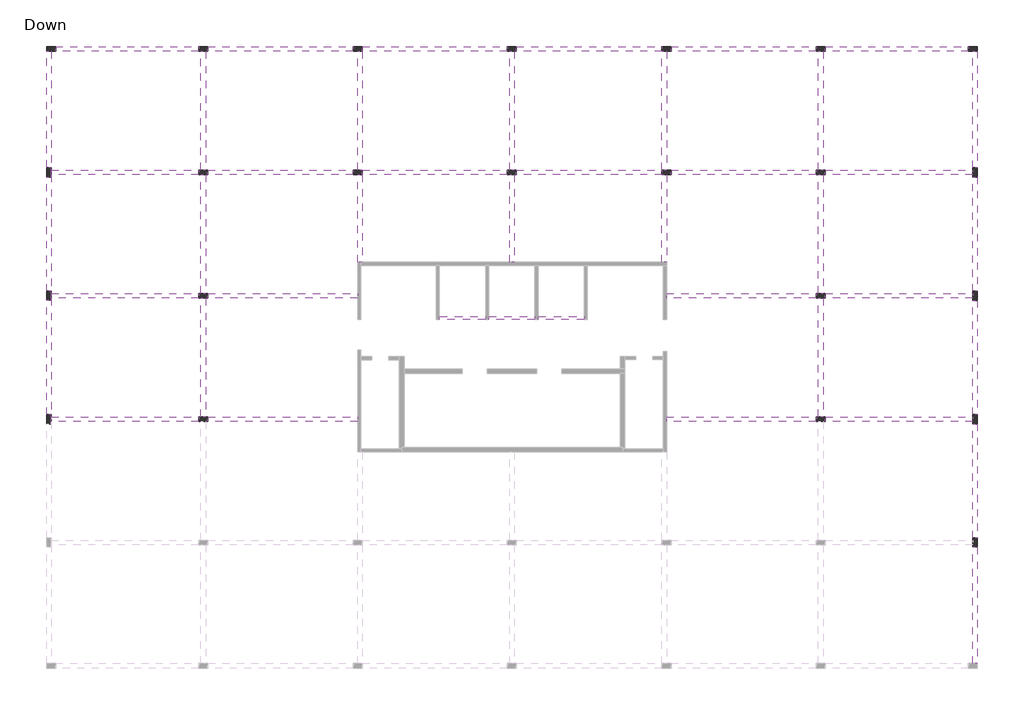
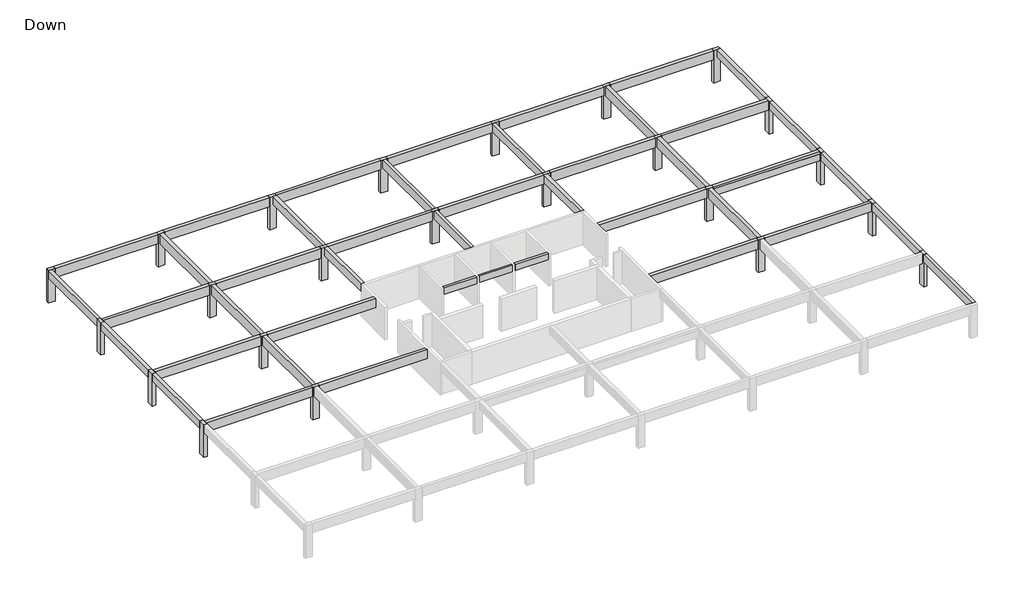
# One storey, part 2 of 2: 43 beams, 23 columns.
# Revit data of these elements (continued)
# Element 19 (IfcBeam, "Concrete Rectengular Beam : 30/85") (continued)
#   Comments = ""
#   Mark = "B27"
#   SOFiSTiK_AMG_Comments = ""
#   SOFiSTiK_AMG_Scheduled = yes
#   SOFiSTiK_AMG_Adjusted = yes
#   Structural Material = Concrete
#   Phase Created = New Construction
#   Materials on its faces: "Concrete"
# Element 20 (IfcBeam, "Concrete Rectengular Beam : 30/85")
#   Comments = ""
#   Mark = "B28"
#   SOFiSTiK_AMG_Comments = ""
#   SOFiSTiK_AMG_Scheduled = yes
#   SOFiSTiK_AMG_Adjusted = yes
#   Structural Material = Concrete
#   Phase Created = New Construction
#   Materials on its faces: "Concrete"
# Element 21 (IfcBeam, "Concrete Rectengular Beam : 30/85")
#   Comments = ""
#   Mark = "B29"
#   SOFiSTiK_AMG_Comments = ""
#   SOFiSTiK_AMG_Scheduled = yes
#   SOFiSTiK_AMG_Adjusted = yes
#   Structural Material = Concrete
#   Phase Created = New Construction
#   Materials on its faces: "Concrete"
# Element 22 (IfcBeam, "Concrete Rectengular Beam : 30/85")
#   Comments = ""
#   Mark = "B30"
#   SOFiSTiK_AMG_Comments = ""
#   SOFiSTiK_AMG_Scheduled = yes
#   SOFiSTiK_AMG_Adjusted = yes
#   Structural Material = Concrete
#   Phase Created = New Construction
#   Materials on its faces: "Concrete"
# Element 23 (IfcBeam, "Concrete Rectengular Beam : 30/85")
#   Comments = ""
#   Mark = "B31"
#   SOFiSTiK_AMG_Comments = ""
#   SOFiSTiK_AMG_Scheduled = yes
#   SOFiSTiK_AMG_Adjusted = yes
#   Structural Material = Concrete
#   Phase Created = New Construction
#   Materials on its faces: "Concrete"
# Element 24 (IfcBeam, "Concrete Rectengular Beam : 30/85")
#   Comments = ""
#   Mark = "B38"
#   SOFiSTiK_AMG_Comments = ""
#   SOFiSTiK_AMG_Scheduled = yes
#   SOFiSTiK_AMG_Adjusted = yes
#   Structural Material = Concrete
#   Phase Created = New Construction
#   Materials on its faces: "Concrete"
# Element 25 (IfcBeam, "Concrete Rectengular Beam : 30/85")
#   Comments = ""
#   Mark = "B39"
#   SOFiSTiK_AMG_Comments = ""
#   SOFiSTiK_AMG_Scheduled = yes
#   SOFiSTiK_AMG_Adjusted = yes
#   Structural Material = Concrete
#   Phase Created = New Construction
#   Materials on its faces: "Concrete"
# Element 26 (IfcBeam, "Concrete Rectengular Beam : 30/85")
#   Comments = ""
#   Mark = "B40"
#   SOFiSTiK_AMG_Comments = ""
#   SOFiSTiK_AMG_Scheduled = yes
#   SOFiSTiK_AMG_Adjusted = yes
#   Structural Material = Concrete
#   Phase Created = New Construction
#   Materials on its faces: "Concrete"
# Element 27 (IfcBeam, "Concrete Rectengular Beam : 30/85")
#   Comments = ""
#   Mark = "B41"
#   SOFiSTiK_AMG_Comments = ""
#   SOFiSTiK_AMG_Scheduled = yes
#   SOFiSTiK_AMG_Adjusted = yes
#   Structural Material = Concrete
#   Phase Created = New Construction
#   Materials on its faces: "Concrete"
# Element 28 (IfcBeam, "Concrete Rectengular Beam : 30/85")
#   Comments = ""
#   Mark = "B42"
#   SOFiSTiK_AMG_Comments = ""
#   SOFiSTiK_AMG_Scheduled = yes
#   SOFiSTiK_AMG_Adjusted = yes
#   Structural Material = Concrete
#   Phase Created = New Construction
#   Materials on its faces: "Concrete"
# Element 29 (IfcBeam, "Concrete Rectengular Beam : 30/85")
#   Comments = ""
#   Mark = "B43"
#   SOFiSTiK_AMG_Comments = ""
#   SOFiSTiK_AMG_Scheduled = yes
#   SOFiSTiK_AMG_Adjusted = yes
#   Structural Material = Concrete
#   Phase Created = New Construction
#   Materials on its faces: "Concrete"
# Element 30 (IfcBeam, "Concrete Rectengular Beam : 30/85")
#   Comments = ""
#   Mark = "B44"
#   SOFiSTiK_AMG_Comments = ""
#   SOFiSTiK_AMG_Scheduled = yes
#   SOFiSTiK_AMG_Adjusted = yes
#   Structural Material = Concrete
#   Phase Created = New Construction
#   Materials on its faces: "Concrete"
# Element 31 (IfcBeam, "Concrete Rectengular Beam : 30/85")
#   Comments = ""
#   Mark = "B45"
#   SOFiSTiK_AMG_Comments = ""
#   SOFiSTiK_AMG_Scheduled = yes
#   SOFiSTiK_AMG_Adjusted = yes
#   Structural Material = Concrete
#   Phase Created = New Construction
#   Materials on its faces: "Concrete"
# Element 32 (IfcBeam, "Concrete Rectengular Beam : 30/90")
#   Comments = ""
#   Mark = "B52"
#   SOFiSTiK_AMG_Comments = ""
#   SOFiSTiK_AMG_Scheduled = yes
#   SOFiSTiK_AMG_Adjusted = yes
#   Structural Material = Concrete
#   Phase Created = New Construction
#   Materials on its faces: "Concrete"
# Element 33 (IfcBeam, "Concrete Rectengular Beam : 30/90")
#   Comments = ""
#   Mark = "B53"
#   SOFiSTiK_AMG_Comments = ""
#   SOFiSTiK_AMG_Scheduled = yes
#   SOFiSTiK_AMG_Adjusted = yes
#   Structural Material = Concrete
#   Phase Created = New Construction
#   Materials on its faces: "Concrete"
# Element 34 (IfcBeam, "Concrete Rectengular Beam : 30/90")
#   Comments = ""
#   Mark = "B54"
#   SOFiSTiK_AMG_Comments = ""
#   SOFiSTiK_AMG_Scheduled = yes
#   SOFiSTiK_AMG_Adjusted = yes
#   Structural Material = Concrete
#   Phase Created = New Construction
#   Materials on its faces: "Concrete"
# Element 35 (IfcBeam, "Concrete Rectengular Beam : 30/90")
#   Comments = ""
#   Mark = "B55"
#   SOFiSTiK_AMG_Comments = ""
#   SOFiSTiK_AMG_Scheduled = yes
#   SOFiSTiK_AMG_Adjusted = yes
#   Structural Material = Concrete
#   Phase Created = New Construction
#   Materials on its faces: "Concrete"
# Element 36 (IfcBeam, "Concrete Rectengular Beam : 30/90")
#   Comments = ""
#   Mark = "B56"
#   SOFiSTiK_AMG_Comments = ""
#   SOFiSTiK_AMG_Scheduled = yes
#   SOFiSTiK_AMG_Adjusted = yes
#   Structural Material = Concrete
#   Phase Created = New Construction
#   Materials on its faces: "Concrete"
# Element 37 (IfcBeam, "Concrete Rectengular Beam : 30/90")
#   Comments = ""
#   Mark = "B57"
#   SOFiSTiK_AMG_Comments = ""
#   SOFiSTiK_AMG_Scheduled = yes
#   SOFiSTiK_AMG_Adjusted = yes
#   Structural Material = Concrete
#   Phase Created = New Construction
#   Materials on its faces: "Concrete"
# Element 38 (IfcBeam, "Concrete Rectengular Beam : 30/90")
#   Comments = ""
#   Mark = "B58"
#   SOFiSTiK_AMG_Comments = ""
#   SOFiSTiK_AMG_Scheduled = yes
#   SOFiSTiK_AMG_Adjusted = yes
#   Structural Material = Concrete
#   Phase Created = New Construction
#   Materials on its faces: "Concrete"
# Element 39 (IfcBeam, "Concrete Rectengular Beam : 30/90")
#   Comments = ""
#   Mark = "B59"
#   SOFiSTiK_AMG_Comments = ""
#   SOFiSTiK_AMG_Scheduled = yes
#   SOFiSTiK_AMG_Adjusted = yes
#   Structural Material = Concrete
#   Phase Created = New Construction
#   Materials on its faces: "Concrete"
# Element 40 (IfcBeam, "Concrete Rectengular Beam : 30/90")
#   Comments = ""
#   Mark = "B60"
#   SOFiSTiK_AMG_Comments = ""
#   SOFiSTiK_AMG_Scheduled = yes
#   SOFiSTiK_AMG_Adjusted = yes
#   Structural Material = Concrete
#   Phase Created = New Construction
#   Materials on its faces: "Concrete"
# Element 41 (IfcBeam, "Concrete Rectengular Beam : 30/90")
#   Comments = ""
#   Mark = "B63"
#   SOFiSTiK_AMG_Comments = ""
#   SOFiSTiK_AMG_Scheduled = yes
#   SOFiSTiK_AMG_Adjusted = yes
#   Structural Material = Concrete
#   Phase Created = New Construction
#   Materials on its faces: "Concrete"
# Element 42 (IfcBeam, "Concrete Rectengular Beam : 30/90")
#   Comments = ""
#   Mark = "B64"
#   SOFiSTiK_AMG_Comments = ""
#   SOFiSTiK_AMG_Scheduled = yes
#   SOFiSTiK_AMG_Adjusted = yes
#   Structural Material = Concrete
#   Phase Created = New Construction
#   Materials on its faces: "Concrete"
# Element 43 (IfcBeam, "Concrete Rectengular Beam : 30/90")
#   Comments = ""
#   Mark = "B65"
#   SOFiSTiK_AMG_Comments = ""
#   SOFiSTiK_AMG_Scheduled = yes
#   SOFiSTiK_AMG_Adjusted = yes
#   Structural Material = Concrete
#   Phase Created = New Construction
#   Materials on its faces: "Concrete"
# Element 44 (IfcColumn, "Concrete Rectengular Column : 30/60")
#   Comments = ""
#   Mark = "C1"
#   SOFiSTiK_AMG_Comments = ""
#   SOFiSTiK_AMG_Scheduled = yes
#   SOFiSTiK_AMG_Adjusted = yes
#   Structural Material = Concrete
#   Phase Created = New Construction
#   Materials on its faces: "Concrete"
# Element 45 (IfcColumn, "Concrete Rectengular Column : 30/60")
#   Comments = ""
#   Mark = "C2"
#   SOFiSTiK_AMG_Comments = ""
#   SOFiSTiK_AMG_Scheduled = yes
#   SOFiSTiK_AMG_Adjusted = yes
#   Structural Material = Concrete
#   Phase Created = New Construction
#   Materials on its faces: "Concrete"
# Element 46 (IfcColumn, "Concrete Rectengular Column : 30/60")
#   Comments = ""
#   Mark = "C4"
#   SOFiSTiK_AMG_Comments = ""
#   SOFiSTiK_AMG_Scheduled = yes
#   SOFiSTiK_AMG_Adjusted = yes
#   Structural Material = Concrete
#   Phase Created = New Construction
#   Materials on its faces: "Concrete"
# Element 47 (IfcColumn, "Concrete Rectengular Column : 30/60")
#   Comments = ""
#   Mark = "C5"
#   SOFiSTiK_AMG_Comments = ""
#   SOFiSTiK_AMG_Scheduled = yes
#   SOFiSTiK_AMG_Adjusted = yes
#   Structural Material = Concrete
#   Phase Created = New Construction
#   Materials on its faces: "Concrete"
# Element 48 (IfcColumn, "Concrete Rectengular Column : 30/60")
#   Comments = ""
#   Mark = "C6"
#   SOFiSTiK_AMG_Comments = ""
#   SOFiSTiK_AMG_Scheduled = yes
#   SOFiSTiK_AMG_Adjusted = yes
#   Structural Material = Concrete
#   Phase Created = New Construction
#   Materials on its faces: "Concrete"
# Element 49 (IfcColumn, "Concrete Rectengular Column : 30/60")
#   Comments = ""
#   Mark = "C9"
#   SOFiSTiK_AMG_Comments = ""
#   SOFiSTiK_AMG_Scheduled = yes
#   SOFiSTiK_AMG_Adjusted = yes
#   Structural Material = Concrete
#   Phase Created = New Construction
#   Materials on its faces: "Concrete"
# Element 50 (IfcColumn, "Concrete Rectengular Column : 30/60")
#   Comments = ""
#   Mark = "C10"
#   SOFiSTiK_AMG_Comments = ""
#   SOFiSTiK_AMG_Scheduled = yes
#   SOFiSTiK_AMG_Adjusted = yes
#   Structural Material = Concrete
#   Phase Created = New Construction
#   Materials on its faces: "Concrete"
# Element 51 (IfcColumn, "Concrete Rectengular Column : 30/60")
#   Comments = ""
#   Mark = "C11"
#   SOFiSTiK_AMG_Comments = ""
#   SOFiSTiK_AMG_Scheduled = yes
#   SOFiSTiK_AMG_Adjusted = yes
#   Structural Material = Concrete
#   Phase Created = New Construction
#   Materials on its faces: "Concrete"
# Element 52 (IfcColumn, "Concrete Rectengular Column : 30/60")
#   Comments = ""
#   Mark = "C12"
#   SOFiSTiK_AMG_Comments = ""
#   SOFiSTiK_AMG_Scheduled = yes
#   SOFiSTiK_AMG_Adjusted = yes
#   Structural Material = Concrete
#   Phase Created = New Construction
#   Materials on its faces: "Concrete"
# Element 53 (IfcColumn, "Concrete Rectengular Column : 30/60")
#   Comments = ""
#   Mark = "C13"
#   SOFiSTiK_AMG_Comments = ""
#   SOFiSTiK_AMG_Scheduled = yes
#   SOFiSTiK_AMG_Adjusted = yes
#   Structural Material = Concrete
#   Phase Created = New Construction
#   Materials on its faces: "Concrete"
# Element 54 (IfcColumn, "Concrete Rectengular Column : 30/60")
#   Comments = ""
#   Mark = "C16"
#   SOFiSTiK_AMG_Comments = ""
#   SOFiSTiK_AMG_Scheduled = yes
#   SOFiSTiK_AMG_Adjusted = yes
#   Structural Material = Concrete
#   Phase Created = New Construction
#   Materials on its faces: "Concrete"
# Element 55 (IfcColumn, "Concrete Rectengular Column : 30/60")
#   Comments = ""
#   Mark = "C18"
#   SOFiSTiK_AMG_Comments = ""
#   SOFiSTiK_AMG_Scheduled = yes
#   SOFiSTiK_AMG_Adjusted = yes
#   Structural Material = Concrete
#   Phase Created = New Construction
#   Materials on its faces: "Concrete"
# Element 56 (IfcColumn, "Concrete Rectengular Column : 30/60")
#   Comments = ""
#   Mark = "C19"
#   SOFiSTiK_AMG_Comments = ""
#   SOFiSTiK_AMG_Scheduled = yes
#   SOFiSTiK_AMG_Adjusted = yes
#   Structural Material = Concrete
#   Phase Created = New Construction
#   Materials on its faces: "Concrete"
# Element 57 (IfcColumn, "Concrete Rectengular Column : 30/60")
#   Comments = ""
#   Mark = "C20"
#   SOFiSTiK_AMG_Comments = ""
#   SOFiSTiK_AMG_Scheduled = yes
#   SOFiSTiK_AMG_Adjusted = yes
#   Structural Material = Concrete
#   Phase Created = New Construction
#   Materials on its faces: "Concrete"
# Element 58 (IfcColumn, "Concrete Rectengular Column : 30/60")
#   Comments = ""
#   Mark = "C21"
#   SOFiSTiK_AMG_Comments = ""
#   SOFiSTiK_AMG_Scheduled = yes
#   SOFiSTiK_AMG_Adjusted = yes
#   Structural Material = Concrete
#   Phase Created = New Construction
#   Materials on its faces: "Concrete"
# Element 59 (IfcColumn, "Concrete Rectengular Column : 30/60")
#   Comments = ""
#   Mark = "C22"
#   SOFiSTiK_AMG_Comments = ""
#   SOFiSTiK_AMG_Scheduled = yes
#   SOFiSTiK_AMG_Adjusted = yes
#   Structural Material = Concrete
#   Phase Created = New Construction
#   Materials on its faces: "Concrete"
# Element 60 (IfcColumn, "Concrete Rectengular Column : 30/60")
#   Comments = ""
#   Mark = "C28"
#   SOFiSTiK_AMG_Comments = ""
#   SOFiSTiK_AMG_Scheduled = yes
#   SOFiSTiK_AMG_Adjusted = yes
#   Structural Material = Concrete
#   Phase Created = New Construction
#   Materials on its faces: "Concrete"
# Element 61 (IfcColumn, "Concrete Rectengular Column : 30/60")
#   Comments = ""
#   Mark = "C29"
#   SOFiSTiK_AMG_Comments = ""
#   SOFiSTiK_AMG_Scheduled = yes
#   SOFiSTiK_AMG_Adjusted = yes
#   Structural Material = Concrete
#   Phase Created = New Construction
#   Materials on its faces: "Concrete"
# Element 62 (IfcColumn, "Concrete Rectengular Column : 30/60")
#   Comments = ""
#   Mark = "C30"
#   SOFiSTiK_AMG_Comments = ""
#   SOFiSTiK_AMG_Scheduled = yes
#   SOFiSTiK_AMG_Adjusted = yes
#   Structural Material = Concrete
#   Phase Created = New Construction
#   Materials on its faces: "Concrete"
# Element 63 (IfcColumn, "Concrete Rectengular Column : 30/60")
#   Comments = ""
#   Mark = "C31"
#   SOFiSTiK_AMG_Comments = ""
#   SOFiSTiK_AMG_Scheduled = yes
#   SOFiSTiK_AMG_Adjusted = yes
#   Structural Material = Concrete
#   Phase Created = New Construction
#   Materials on its faces: "Concrete"
# Element 64 (IfcColumn, "Concrete Rectengular Column : 30/60")
#   Comments = ""
#   Mark = "C32"
#   SOFiSTiK_AMG_Comments = ""
#   SOFiSTiK_AMG_Scheduled = yes
#   SOFiSTiK_AMG_Adjusted = yes
#   Structural Material = Concrete
#   Phase Created = New Construction
#   Materials on its faces: "Concrete"
# Element 65 (IfcColumn, "Concrete Rectengular Column : 30/60")
#   Comments = ""
#   Mark = "C33"
#   SOFiSTiK_AMG_Comments = ""
#   SOFiSTiK_AMG_Scheduled = yes
#   SOFiSTiK_AMG_Adjusted = yes
#   Structural Material = Concrete
#   Phase Created = New Construction
#   Materials on its faces: "Concrete"
# Element 66 (IfcColumn, "Concrete Rectengular Column : 30/60")
#   Comments = ""
#   Mark = "C34"
#   SOFiSTiK_AMG_Comments = ""
#   SOFiSTiK_AMG_Scheduled = yes
#   SOFiSTiK_AMG_Adjusted = yes
#   Structural Material = Concrete
#   Phase Created = New Construction
#   Materials on its faces: "Concrete"
# Materials
#   "Concrete": class "Concrete", colour RGB 192 192 192, transparency 0, Keynote = "01000", Description = "Cast-in-place concrete", Cost = 0
